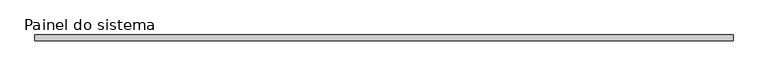
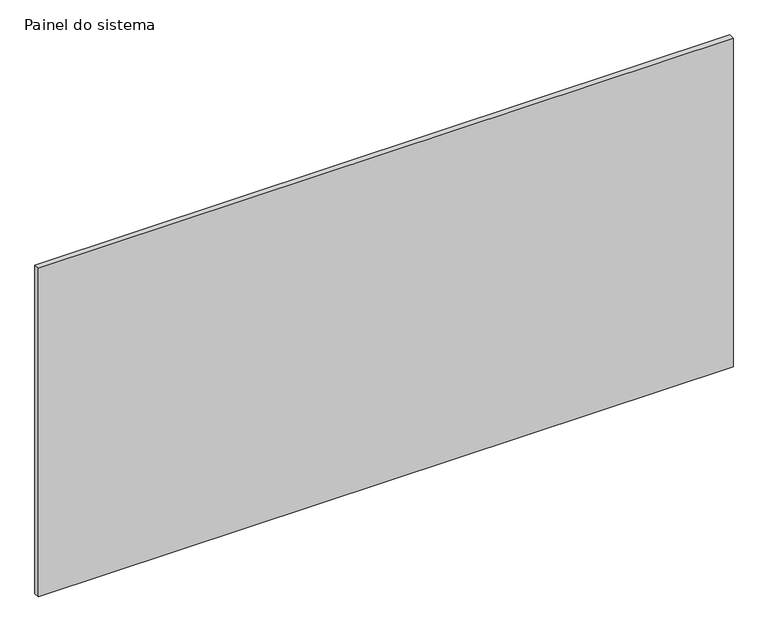
"""IFC4 building model written with IfcOpenShell, lengths in millimetres: plate geometry, Painel do sistema : Envidraçado."""

from ifc_helpers import new_model, si_unit, origin, origin_with_axes, place, context, project, spatial, polyline, outline, extrude, source, transform, mapped, element, save


def painel_do_sistema_b8becc76(model_context):
    return source(origin(), model_context, "Body", "SweptSolid", [
        extrude(outline(polyline([(1499.9999925, 24.5), (-1499.9999925, 24.5), (-1499.9999925, 49.5), (1499.9999925, 49.5), (1499.9999925, 24.5)])), origin_with_axes(), (0.0, 0.0, 1.0), 1500.0),
    ])


if __name__ == "__main__":
    model = new_model("IFC4")
    model_context = context("Model", 3, world=origin())
    ifc_project = project(units=[si_unit("LENGTHUNIT", "METRE", prefix="MILLI")], contexts=[model_context])
    site = spatial("IfcSite", under=ifc_project)
    building = spatial("IfcBuilding", under=site)
    placement = place(None, origin())
    painel_do_sistema_shape = painel_do_sistema_b8becc76(model_context)
    element("IfcPlate", 1, ObjectType="Painel do sistema : Envidraçado", at=placement, inside=building, context=model_context, shape_type="MappedRepresentation", body=[
        mapped(painel_do_sistema_shape, transform((0.0, 0.0, 0.0), x_axis=(1.0, 0.0, 0.0), y_axis=(0.0, 1.0, 0.0), z_axis=(0.0, 0.0, 1.0))),
    ])
    save(model, "model.ifc")

# Revit data of these elements
# Type "Painel do sistema : Envidraçado"
#   Construction Type Id = "GSP4R"
#   Analytic Construction = "Vidraça única Pilkington 1/8 pol"
#   Visual Light Transmittance = 0.9
#   Solar Heat Gain Coefficient = 0.86
#   Heat Transfer Coefficient (U) = 6.7069 W/(m²·K)
# Element 1 (IfcPlate, "Painel do sistema : Envidraçado")
#   Materials on its faces: "Vidro"
# Materials
#   "Vidro": class "Vidro", colour RGB 0 128 192, transparency 0.9, Description = "Vidro de sílica", Cost = 0
